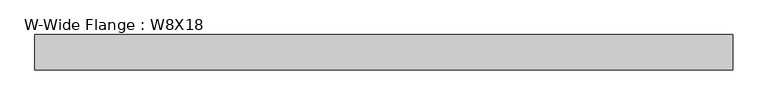
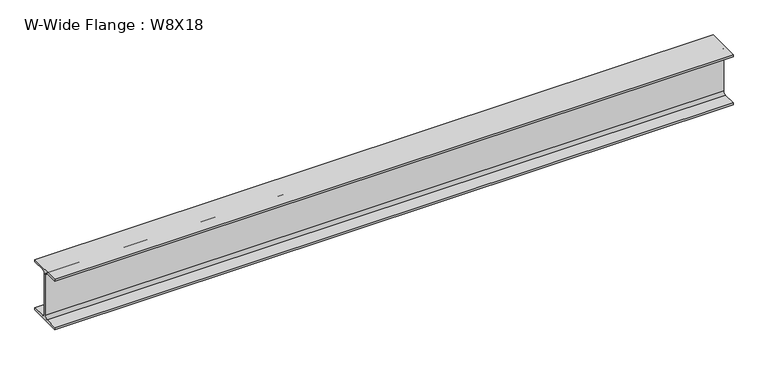
"""IFC4 building model written with IfcOpenShell, lengths in millimetres: beam geometry, W-Wide Flange : W8X18."""

from ifc_helpers import new_model, si_unit, point, frame, frame_2d, origin, place, context, project, spatial, polyline, circle_curve, trimmed, segment, composite_curve, outline, extrude, source, transform, mapped, element, save


def w_wide_flange_w8x18_17d6e70c(model_context):
    return source(origin(), model_context, "Body", "SweptSolid", [
        extrude(outline(composite_curve([segment(polyline([(66.675, -94.996), (66.675, -103.378), (-66.675, -103.378), (-66.675, -94.996), (-15.1765, -94.996)]), True, "CONTINUOUS"), segment(trimmed(circle_curve(frame_2d((-15.1765, -82.7405)), 12.2555), [point((-15.1765, -94.996))], [point((-2.921, -82.7405))], True, "CARTESIAN"), True, "CONTINUOUS"), segment(polyline([(-2.921, -82.7405), (-2.921, 82.7405)]), True, "CONTINUOUS"), segment(trimmed(circle_curve(frame_2d((-15.1765, 82.7405)), 12.2555), [point((-2.921, 82.7405))], [point((-15.1765, 94.996))], True, "CARTESIAN"), True, "CONTINUOUS"), segment(polyline([(-15.1765, 94.996), (-66.675, 94.996), (-66.675, 103.378), (66.675, 103.378), (66.675, 94.996), (15.1765, 94.996)]), True, "CONTINUOUS"), segment(trimmed(circle_curve(frame_2d((15.1765, 82.7405)), 12.2555), [point((15.1765, 94.996))], [point((2.921, 82.7405))], True, "CARTESIAN"), True, "CONTINUOUS"), segment(polyline([(2.921, 82.7405), (2.921, -82.7405)]), True, "CONTINUOUS"), segment(trimmed(circle_curve(frame_2d((15.1765, -82.7405)), 12.2555), [point((2.921, -82.7405))], [point((15.1765, -94.996))], True, "CARTESIAN"), True, "CONTINUOUS"), segment(polyline([(15.1765, -94.996), (66.675, -94.996)]), True, "CONTINUOUS")], self_intersect=False)), frame((-1321.0747268, 0.0, 0.0), z_axis=(1.0, 0.0, 0.0), x_axis=(0.0, 1.0, 0.0)), (0.0, 0.0, 1.0), 2633.9372268),
    ])


if __name__ == "__main__":
    model = new_model("IFC4")
    model_context = context("Model", 3, world=origin())
    ifc_project = project(units=[si_unit("LENGTHUNIT", "METRE", prefix="MILLI")], contexts=[model_context])
    site = spatial("IfcSite", under=ifc_project)
    building = spatial("IfcBuilding", under=site)
    placement = place(None, origin())
    w_wide_flange_w8x18_shape = w_wide_flange_w8x18_17d6e70c(model_context)
    element("IfcBeam", 1, ObjectType="W-Wide Flange : W8X18", at=placement, inside=building, context=model_context, shape_type="MappedRepresentation", body=[
        mapped(w_wide_flange_w8x18_shape, transform((0.0, 0.0, 0.0), x_axis=(1.0, 0.0, 0.0), y_axis=(0.0, 1.0, 0.0), z_axis=(0.0, 0.0, 1.0))),
    ])
    save(model, "model.ifc")

# Revit data of these elements
# Type "W-Wide Flange : W8X18"
#   Assembly Code = "B10"
#   W = 18
#   Length [instance default] = 1524 mm
#   bf = 133.35 mm
#   d = 206.756 mm
#   k = 20.638 mm
#   k2 = 12.256 mm
#   tf = 8.382 mm
#   tw = 5.842 mm
#   A = 0.00339354 m²
#   Structural Material [instance default] = Steel ASTM A992
# Element 1 (IfcBeam, "W-Wide Flange : W8X18")
#   Structural Material = Aluminum, Anodized Red
#   Materials on its faces: "Aluminum, Anodized Red"
# Materials
#   "Steel ASTM A992": class "Metal", colour RGB 128 0 0, transparency 0, Description = "Structural steel 50ksi", Cost = 0
#   "Aluminum, Anodized Red": class "Metal", colour RGB 120 120 120, transparency 0, Description = "Anodized aluminum, red", Cost = 0
